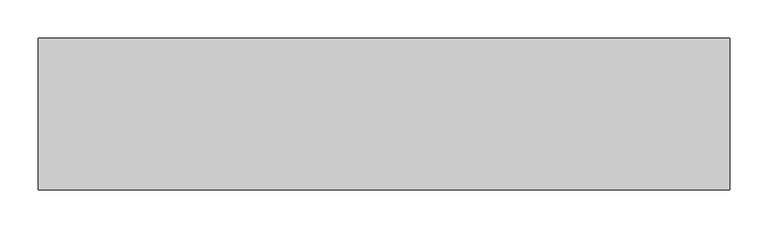
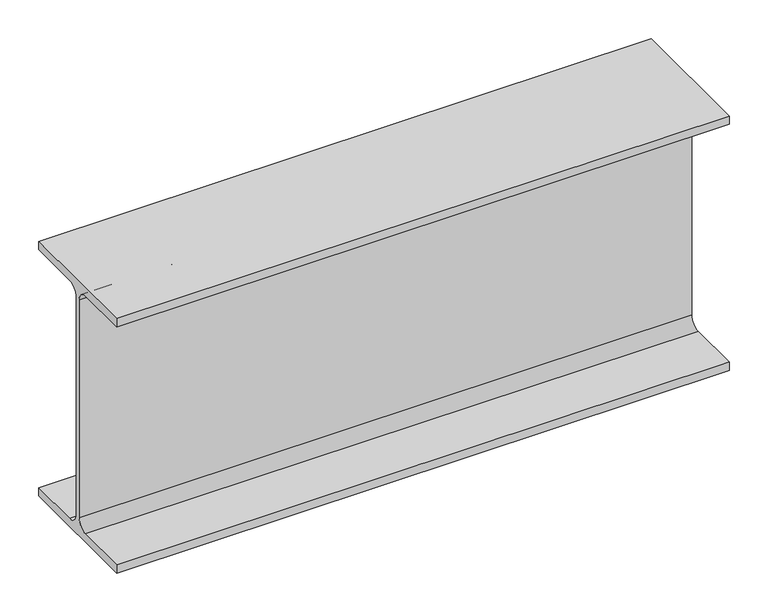
"""IFC4 building model written with IfcOpenShell, lengths in millimetres: beam geometry, Steel Framing_H_KS : H_SB_AR_S02_H-400x200x8x13_SCB1."""

import ifcopenshell
import ifcopenshell.guid

model = None  # the IFC model being written
_history = None  # IfcOwnerHistory: only IFC2X3 demands one
_inside = {}  # id of a spatial element -> (the spatial element, [elements in it])
_under = {}  # id of a project, library or spatial element -> (it, [spatial elements below it])
_declared = {}  # id of a project -> (the project, [libraries it declares])
_typed = {}  # id of a type object -> (the type object, [elements of that type])
_made_of = {}  # id of a material, layer set ... -> (it, [elements and type objects made of it])


def new_model(schema):
    """Start an empty IFC model of exactly this schema.

    Asked for "IFC4X3", IfcOpenShell would pick the latest addendum, in which some entities
    have other attributes; the version numbers below select the first issue.
    IFC2X3 requires an IfcOwnerHistory on every rooted entity: one is made here for all.
    """
    global model, _history
    if schema == "IFC4X3":
        model = ifcopenshell.file(schema_version=(4, 3, 0, 0))
    else:
        model = ifcopenshell.file(schema=schema)
    _inside.clear()
    _under.clear()
    _declared.clear()
    _typed.clear()
    _made_of.clear()
    _history = None
    if model.schema == "IFC2X3":
        org = make("IfcOrganization", Name="unknown")
        user = make(
            "IfcPersonAndOrganization",
            ThePerson=make("IfcPerson", FamilyName="unknown"),
            TheOrganization=org,
        )
        app = make(
            "IfcApplication",
            ApplicationDeveloper=org,
            Version="unknown",
            ApplicationFullName="unknown",
            ApplicationIdentifier="unknown",
        )
        _history = make(
            "IfcOwnerHistory",
            OwningUser=user,
            OwningApplication=app,
            ChangeAction="ADDED",
            CreationDate=0,
        )
    return model


def make(cls, **values):
    """One entity of the class cls with the attributes given. An attribute that is None is left unset."""
    return model.create_entity(
        cls, **{name: value for name, value in values.items() if value is not None}
    )


def rooted(cls, **values):
    """An entity with a GlobalId (a new one), such as an element, a storey or a relation."""
    return make(cls, GlobalId=ifcopenshell.guid.new(), OwnerHistory=_history, **values)


def si_unit(unit_type, name, prefix=None):
    """IfcSIUnit, for example si_unit("LENGTHUNIT", "METRE", prefix="MILLI")."""
    return make("IfcSIUnit", UnitType=unit_type, Prefix=prefix, Name=name)


def assignment(units):
    """IfcUnitAssignment: the units of a project."""
    return None if units is None else make("IfcUnitAssignment", Units=units)


def point(xyz):
    """IfcCartesianPoint."""
    return None if xyz is None else make("IfcCartesianPoint", Coordinates=xyz)


def direction(xyz):
    """IfcDirection."""
    return None if xyz is None else make("IfcDirection", DirectionRatios=xyz)


def frame(location, z_axis=None, x_axis=None):
    """IfcAxis2Placement3D, a coordinate frame: its origin and axes. An axis left out is left unset."""
    return make(
        "IfcAxis2Placement3D",
        Location=point(location),
        Axis=direction(z_axis),
        RefDirection=direction(x_axis),
    )


def frame_2d(location, x_axis=None):
    """IfcAxis2Placement2D, a coordinate frame in the plane: its origin and x axis."""
    return make(
        "IfcAxis2Placement2D", Location=point(location), RefDirection=direction(x_axis)
    )


def origin():
    """The frame at (0, 0, 0) with its axes left unset."""
    return frame((0.0, 0.0, 0.0))


def place(relative_to, where):
    """IfcLocalPlacement: puts the frame where relative to a parent placement (None: the world)."""
    return make(
        "IfcLocalPlacement", PlacementRelTo=relative_to, RelativePlacement=where
    )


def context(
    kind, dimensions, precision=None, world=None, true_north=None, identifier=None
):
    """IfcGeometricRepresentationContext, for example the 3D "Model" context."""
    return make(
        "IfcGeometricRepresentationContext",
        ContextIdentifier=identifier,
        ContextType=kind,
        CoordinateSpaceDimension=dimensions,
        Precision=precision,
        WorldCoordinateSystem=world,
        TrueNorth=true_north,
    )


def project(units=None, contexts=None):
    """IfcProject with its units and contexts."""
    return rooted(
        "IfcProject",
        Name="project",
        RepresentationContexts=contexts,
        UnitsInContext=assignment(units),
    )


def spatial(cls, under=None, at=None, **own):
    """A site, building, storey or space (cls), placed at a placement, below another one or the project."""
    s = rooted(cls, ObjectPlacement=at, **own)
    if under is not None:
        _under.setdefault(under.id(), (under, []))[1].append(s)
    return s


def polyline(points):
    """IfcPolyline through the points."""
    return make("IfcPolyline", Points=[point(p) for p in points])


def circle_curve(where, radius):
    """IfcCircle in the frame where."""
    return make("IfcCircle", Position=where, Radius=radius)


def trimmed(basis, trim1, trim2, sense, master):
    """IfcTrimmedCurve: the piece of a basis curve between two trims."""
    return make(
        "IfcTrimmedCurve",
        BasisCurve=basis,
        Trim1=trim1,
        Trim2=trim2,
        SenseAgreement=sense,
        MasterRepresentation=master,
    )


def segment(curve, same_sense, transition):
    """IfcCompositeCurveSegment."""
    return make(
        "IfcCompositeCurveSegment",
        Transition=transition,
        SameSense=same_sense,
        ParentCurve=curve,
    )


def composite_curve(segments, self_intersect=None):
    """IfcCompositeCurve: segments joined end to end."""
    return make("IfcCompositeCurve", Segments=segments, SelfIntersect=self_intersect)


def outline(outer, holes=None, kind="AREA"):
    """IfcArbitraryClosedProfileDef: a profile drawn as a closed curve; with holes, ...WithVoids."""
    if holes is None:
        return make("IfcArbitraryClosedProfileDef", ProfileType=kind, OuterCurve=outer)
    return make(
        "IfcArbitraryProfileDefWithVoids",
        ProfileType=kind,
        OuterCurve=outer,
        InnerCurves=holes,
    )


def extrude(swept, where, along, depth):
    """IfcExtrudedAreaSolid: the profile swept, set in the frame where, extruded along a direction by depth."""
    return make(
        "IfcExtrudedAreaSolid",
        SweptArea=swept,
        Position=where,
        ExtrudedDirection=direction(along),
        Depth=depth,
    )


def shape(context_of_items, identifier, shape_type, items):
    """IfcShapeRepresentation: the items that make up one representation, for example the "Body"."""
    return make(
        "IfcShapeRepresentation",
        ContextOfItems=context_of_items,
        RepresentationIdentifier=identifier,
        RepresentationType=shape_type,
        Items=items,
    )


def source(mapping_origin, context_of_items, identifier, shape_type, items):
    """IfcRepresentationMap: a shape defined once, which mapped items show again and again."""
    return make(
        "IfcRepresentationMap",
        MappingOrigin=mapping_origin,
        MappedRepresentation=shape(context_of_items, identifier, shape_type, items),
    )


def transform(
    local_origin,
    x_axis=None,
    y_axis=None,
    z_axis=None,
    scale=None,
    scale2=None,
    scale3=None,
    uniform=True,
):
    """IfcCartesianTransformationOperator3D, or its non-uniform kind. x_axis, y_axis, z_axis: its Axis1, 2, 3."""
    if uniform:
        return make(
            "IfcCartesianTransformationOperator3D",
            Axis1=direction(x_axis),
            Axis2=direction(y_axis),
            LocalOrigin=point(local_origin),
            Scale=scale,
            Axis3=direction(z_axis),
        )
    return make(
        "IfcCartesianTransformationOperator3DnonUniform",
        Axis1=direction(x_axis),
        Axis2=direction(y_axis),
        LocalOrigin=point(local_origin),
        Scale=scale,
        Axis3=direction(z_axis),
        Scale2=scale2,
        Scale3=scale3,
    )


def mapped(mapping_source, mapping_target):
    """IfcMappedItem: shows the shape of a source again, moved by a transform."""
    return make(
        "IfcMappedItem", MappingSource=mapping_source, MappingTarget=mapping_target
    )


def made_of(thing, what):
    """Note that an element or type object is made of a material, layer set ...; save() writes the relation."""
    if what is not None:
        _made_of.setdefault(what.id(), (what, []))[1].append(thing)
    return thing


def element(
    cls,
    number,
    at=None,
    inside=None,
    cuts=None,
    type_object=None,
    material=None,
    context=None,
    identifier="Body",
    shape_type=None,
    held_by="IfcProductDefinitionShape",
    body=None,
    shapes=None,
    **own,
):
    """One element of the class cls, such as IfcWall. Its Tag is "e" and its number.

    at: its placement. inside: the storey or other place that contains it. cuts: it is an
    opening in that element (IfcRelVoidsElement). A single representation is given by context,
    identifier, shape_type and body (its items); several are given by shapes. held_by: the class
    of the entity that holds the representations. save() writes the other relations.
    """
    e = rooted(cls, Tag="e%d" % number, ObjectPlacement=at, **own)
    if body is not None:
        shapes = [shape(context, identifier, shape_type, body)]
    if shapes is not None:
        e.Representation = make(held_by, Representations=shapes)
    if inside is not None:
        _inside.setdefault(inside.id(), (inside, []))[1].append(e)
    if cuts is not None:
        rooted(
            "IfcRelVoidsElement", RelatingBuildingElement=cuts, RelatedOpeningElement=e
        )
    if type_object is not None:
        _typed.setdefault(type_object.id(), (type_object, []))[1].append(e)
    return made_of(e, material)


def aggregate(whole, parts):
    """IfcRelAggregates: a whole, such as a stair, and the parts it consists of."""
    return rooted("IfcRelAggregates", RelatingObject=whole, RelatedObjects=parts)


def save(model, path):
    """Write the relations noted so far, then the file.

    IfcRelAggregates (storeys below a building ...), IfcRelContainedInSpatialStructure (elements
    in a storey), IfcRelDefinesByType, IfcRelAssociatesMaterial and IfcRelDeclares: one each for
    every whole, place, type object, material and project.
    """
    for whole, parts in _under.values():
        aggregate(whole, parts)
    for where, things in _inside.values():
        rooted(
            "IfcRelContainedInSpatialStructure",
            RelatedElements=things,
            RelatingStructure=where,
        )
    for kind, things in _typed.values():
        rooted("IfcRelDefinesByType", RelatedObjects=things, RelatingType=kind)
    for what, things in _made_of.values():
        rooted("IfcRelAssociatesMaterial", RelatedObjects=things, RelatingMaterial=what)
    for by, libraries in _declared.values():
        rooted("IfcRelDeclares", RelatingContext=by, RelatedDefinitions=libraries)
    model.write(path)


def beam_29f4eb64(model_context):
    return source(origin(), model_context, "Body", "SweptSolid", [
        extrude(outline(composite_curve([segment(polyline([(-100.0, -187.0), (-20.0, -187.0)]), True, "CONTINUOUS"), segment(trimmed(circle_curve(frame_2d((-20.0, -171.0)), 16.0), [point((-20.0, -187.0))], [point((-4.0, -171.0))], True, "CARTESIAN"), True, "CONTINUOUS"), segment(polyline([(-4.0, -171.0), (-4.0, 171.0)]), True, "CONTINUOUS"), segment(trimmed(circle_curve(frame_2d((-20.0, 171.0)), 16.0), [point((-4.0, 171.0))], [point((-20.0, 187.0))], True, "CARTESIAN"), True, "CONTINUOUS"), segment(polyline([(-20.0, 187.0), (-100.0, 187.0), (-100.0, 200.0), (100.0, 200.0), (100.0, 187.0), (20.0, 187.0)]), True, "CONTINUOUS"), segment(trimmed(circle_curve(frame_2d((20.0, 171.0)), 16.0), [point((20.0, 187.0))], [point((4.0, 171.0))], True, "CARTESIAN"), True, "CONTINUOUS"), segment(polyline([(4.0, 171.0), (4.0, -171.0)]), True, "CONTINUOUS"), segment(trimmed(circle_curve(frame_2d((20.0, -171.0)), 16.0), [point((4.0, -171.0))], [point((20.0, -187.0))], True, "CARTESIAN"), True, "CONTINUOUS"), segment(polyline([(20.0, -187.0), (100.0, -187.0), (100.0, -200.0), (-100.0, -200.0), (-100.0, -187.0)]), True, "CONTINUOUS")], self_intersect=False)), frame((-380.0, 0.0, 0.0), z_axis=(1.0, 0.0, 0.0), x_axis=(0.0, 1.0, 0.0)), (0.0, 0.0, 1.0), 910.0),
    ])


if __name__ == "__main__":
    model = new_model("IFC4")
    model_context = context("Model", 3, world=origin())
    ifc_project = project(units=[si_unit("LENGTHUNIT", "METRE", prefix="MILLI")], contexts=[model_context])
    site = spatial("IfcSite", under=ifc_project)
    building = spatial("IfcBuilding", under=site)
    placement = place(None, origin())
    beam_shape = beam_29f4eb64(model_context)
    element("IfcBeam", 1, ObjectType="Steel Framing_H_KS : H_SB_AR_S02_H-400x200x8x13_SCB1", at=placement, inside=building, context=model_context, shape_type="MappedRepresentation", body=[
        mapped(beam_shape, transform((0.0, 0.0, 0.0), x_axis=(1.0, 0.0, 0.0), y_axis=(0.0, 1.0, 0.0), z_axis=(0.0, 0.0, 1.0))),
    ])
    save(model, "model.ifc")

# Revit data of these elements
# Type "Steel Framing_H_KS : H_SB_AR_S02_H-400x200x8x13_SCB1"
#   Type Comments = "MAIN"
#   Type Mark = "SCB1"
#   H_SectionID = "H-400x200x8x13"
#   H_Ratio for Additional Steel Plate = 0.2
#   Width = 20.0 cm
#   Web Thickness = 0.8 cm
#   Web Fillet = 1.6 cm
#   Warping Constant = 649000.0 cm⁶
#   Torsional Moment of Inertia = 35.8981 cm⁴
#   Section Area = 84.12 cm²
#   Plastic Modulus weak axis = 268.0 cm³
#   Plastic Modulus strong axis = 1330.0 cm³
#   Perimeter = 1.56 m²/m
#   Nominal Weight = 66.00 kgf/m
#   Moment of Inertia weak axis = 1740.00 cm⁴
#   Moment of Inertia strong axis = 23700.00 cm⁴
#   Height = 40.0 cm
#   Flange Thickness = 1.3 cm
#   Elastic Modulus weak axis = 174.0 cm³
#   Elastic Modulus strong axis = 1190.0 cm³
#   Centroid Vertical = 20.0 cm
#   Centroid Horizontal = 10.0 cm
#   Bolt Spacing = 8.89 cm
#   Length [instance default] = 1500 mm
#   Structural Material [instance default] = Steel, 45-345
#   Section Name Key = ""
#   Assembly Code = ""
# Element 1 (IfcBeam, "Steel Framing_H_KS : H_SB_AR_S02_H-400x200x8x13_SCB1")
#   Materials on its faces: "Steel, 45-345"
# Materials
#   "Steel, 45-345": class "Metal", colour RGB 189 187 185, transparency 0, Description = "Steel 345 MPa", Cost = 0
